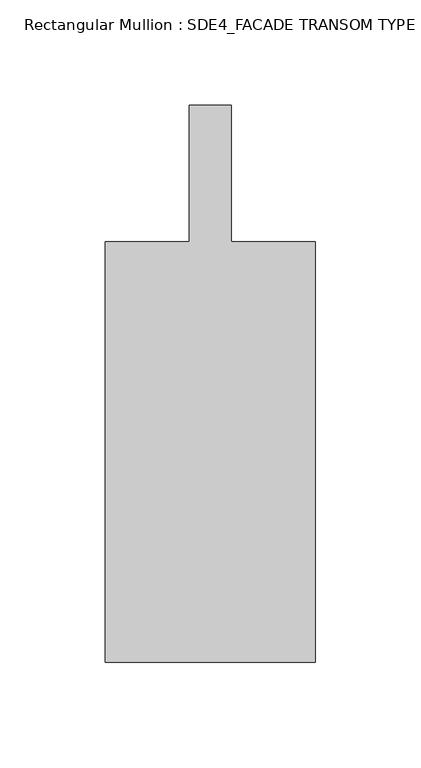
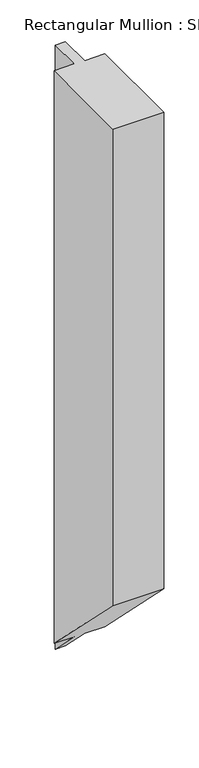
"""IFC4 building model written with IfcOpenShell, lengths in millimetres: member geometry, Rectangular Mullion : SDE4_FACADE TRANSOM TYPE 2."""

from ifc_helpers import new_model, si_unit, origin, place, context, project, spatial, faceted_brep, source, transform, mapped, element, save


def rectangular_mullion_sde4_facade_transom_type_2_69a8b3ca(model_context):
    return source(origin(), model_context, "Body", "Brep", [
        faceted_brep([(50.0, -132.5, 0.0), (50.0, 67.5, 0.0), (10.0, 67.5, 0.0), (10.0, 132.5, 0.0), (-10.0, 132.5, 0.0), (-10.0, 67.5, 0.0), (-50.0, 67.5, 0.0), (-50.0, -132.5, 0.0), (50.0, -132.5, -990.0), (50.0, 67.5, -1190.0), (10.0, 67.5, -1190.0), (10.0, 132.5, -1255.0), (-10.0, 132.5, -1255.0), (-10.0, 67.5, -1190.0), (-50.0, 67.5, -1190.0), (-50.0, -132.5, -990.0)], [[[0, 1, 2, 3, 4, 5, 6, 7]], [[1, 0, 8, 9]], [[2, 1, 9, 10]], [[3, 2, 10, 11]], [[4, 3, 11, 12]], [[5, 4, 12, 13]], [[6, 5, 13, 14]], [[7, 6, 14, 15]], [[0, 7, 15, 8]], [[8, 15, 14, 13, 12, 11, 10, 9]]]),
    ])


if __name__ == "__main__":
    model = new_model("IFC4")
    model_context = context("Model", 3, world=origin())
    ifc_project = project(units=[si_unit("LENGTHUNIT", "METRE", prefix="MILLI")], contexts=[model_context])
    site = spatial("IfcSite", under=ifc_project)
    building = spatial("IfcBuilding", under=site)
    placement = place(None, origin())
    rectangular_mullion_sde4_facade_transom_type_2_shape = rectangular_mullion_sde4_facade_transom_type_2_69a8b3ca(model_context)
    element("IfcMember", 1, ObjectType="Rectangular Mullion : SDE4_FACADE TRANSOM TYPE 2", at=placement, inside=building, context=model_context, shape_type="MappedRepresentation", body=[
        mapped(rectangular_mullion_sde4_facade_transom_type_2_shape, transform((0.0, 0.0, 0.0), x_axis=(1.0, 0.0, 0.0), y_axis=(0.0, 1.0, 0.0), z_axis=(0.0, 0.0, 1.0))),
    ])
    save(model, "model.ifc")

# Revit data of these elements
# Type "Rectangular Mullion : SDE4_FACADE TRANSOM TYPE 2"
#   built-in parameter 1007322 = 0.869423 (stored number, unit not read)
#   built-in parameter 1007321 = 0.164042 (stored number, unit not read)
#   built-in parameter 1007320 = 0.164042 (stored number, unit not read)
